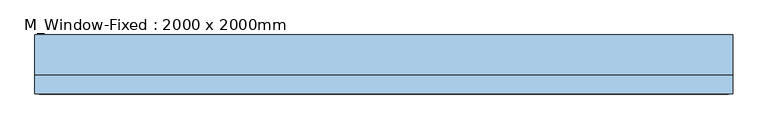
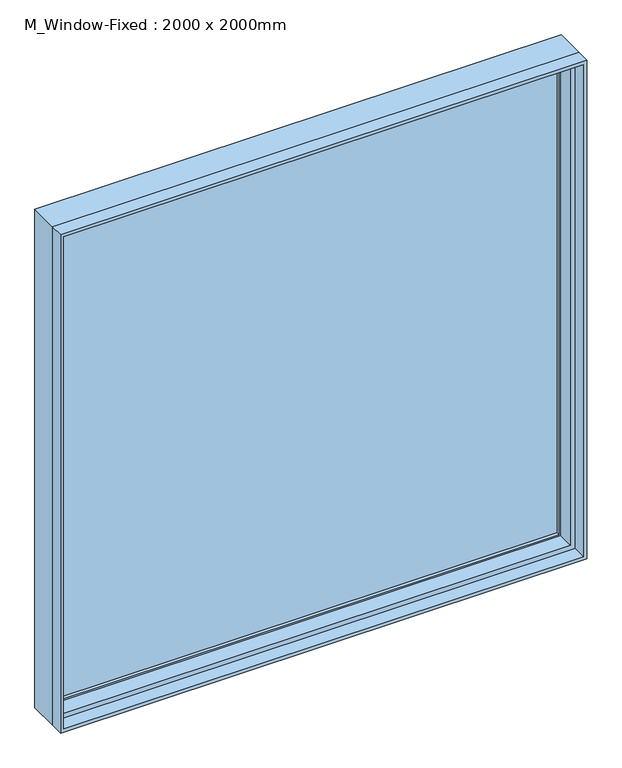
"""IFC4 building model written with IfcOpenShell, lengths in millimetres: window geometry, M_Window-Fixed : 2000 x 2000mm."""

from ifc_helpers import new_model, si_unit, frame, origin, place, context, project, spatial, polyline, outline, extrude, faceted_brep, source, transform, mapped, element, save


def m_window_fixed_2000_x_2000mm_1dfd0f54(model_context):
    return source(origin(), model_context, "Body", "SolidModel", [
        faceted_brep([(1000.0, -20.25, 2900.0), (1000.0, 94.05, 2900.0), (-1000.0, 94.05, 2900.0), (-1000.0, -20.25, 2900.0), (-1000.0, 94.05, 900.0), (-1000.0, -20.25, 900.0), (1000.0, 94.05, 900.0), (1000.0, -20.25, 900.0), (968.25, -20.25, 2868.25), (968.25, -20.25, 931.75), (-968.25, -20.25, 931.75), (-968.25, -20.25, 2868.25), (-987.3, 94.05, 2887.3), (-987.3, 94.05, 912.7), (987.3, 94.05, 912.7), (987.3, 94.05, 2887.3), (968.25, 43.25, 2868.25), (-968.25, 43.25, 2868.25), (987.3, 43.25, 2887.3), (-987.3, 43.25, 2887.3), (-968.25, 43.25, 931.75), (-987.3, 43.25, 912.7), (968.25, 43.25, 931.75), (987.3, 43.25, 912.7)], [[[0, 1, 2, 3]], [[3, 2, 4, 5]], [[5, 4, 6, 7]], [[3, 5, 7, 0], [8, 9, 10, 11]], [[7, 6, 1, 0]], [[1, 6, 4, 2], [12, 13, 14, 15]], [[16, 8, 11, 17]], [[15, 18, 19, 12]], [[17, 11, 10, 20]], [[12, 19, 21, 13]], [[20, 10, 9, 22]], [[13, 21, 23, 14]], [[22, 9, 8, 16]], [[18, 23, 21, 19], [17, 20, 22, 16]], [[14, 23, 18, 15]]]),
        extrude(outline(polyline([(2900.0, -1000.0), (900.0, -1000.0), (900.0, 1000.0), (2900.0, 1000.0), (2900.0, -1000.0)]), holes=[polyline([(2887.3, 987.3), (912.7, 987.3), (912.7, -987.3), (2887.3, -987.3), (2887.3, 987.3)])]), frame((0.0, -75.0, 0.0), z_axis=(0.0, 1.0, 0.0), x_axis=(0.0, 0.0, 1.0)), (0.0, 0.0, 1.0), 54.75),
        extrude(outline(polyline([(912.7, 987.3), (2887.3, 987.3), (2887.3, -987.3), (912.7, -987.3), (912.7, 987.3)]), holes=[polyline([(938.1, -961.9), (2861.9, -961.9), (2861.9, 961.9), (938.1, 961.9), (938.1, -961.9)])]), frame((0.0, 43.25, 0.0), z_axis=(0.0, 1.0, 0.0), x_axis=(0.0, 0.0, 1.0)), (0.0, 0.0, 1.0), 44.45),
        extrude(outline(polyline([(961.9, 75.0), (961.9, 68.65), (-961.9, 68.65), (-961.9, 75.0), (961.9, 75.0)])), frame((0.0, 0.0, 938.1), z_axis=(0.0, 0.0, 1.0), x_axis=(1.0, 0.0, 0.0)), (0.0, 0.0, 1.0), 1923.8),
        extrude(outline(polyline([(-961.9, 55.95), (-961.9, 62.3), (961.9, 62.3), (961.9, 55.95), (-961.9, 55.95)])), frame((0.0, 0.0, 938.1), z_axis=(0.0, 0.0, 1.0), x_axis=(1.0, 0.0, 0.0)), (0.0, 0.0, 1.0), 1923.8),
    ])


if __name__ == "__main__":
    model = new_model("IFC4")
    model_context = context("Model", 3, world=origin())
    ifc_project = project(units=[si_unit("LENGTHUNIT", "METRE", prefix="MILLI")], contexts=[model_context])
    site = spatial("IfcSite", under=ifc_project)
    building = spatial("IfcBuilding", under=site)
    placement = place(None, origin())
    m_window_fixed_2000_x_2000mm_shape = m_window_fixed_2000_x_2000mm_1dfd0f54(model_context)
    element("IfcWindow", 1, ObjectType="M_Window-Fixed : 2000 x 2000mm", at=placement, inside=building, context=model_context, shape_type="MappedRepresentation", body=[
        mapped(m_window_fixed_2000_x_2000mm_shape, transform((0.0, 0.0, 0.0), x_axis=(1.0, 0.0, 0.0), y_axis=(0.0, 1.0, 0.0), z_axis=(0.0, 0.0, 1.0))),
    ])
    save(model, "model.ifc")

# Revit data of these elements
# Type "M_Window-Fixed : 2000 x 2000mm"
#   Type Mark = "40"
#   Fire Rating = "0.5h"
#   Assembly Code = "B2020100"
#   Analytic Construction = "Double glazing - domestic"
#   Window Inset [instance default] = 0 mm
#   Wall Thickness [instance default] = 150 mm
#   Visual Light Transmittance = 0.81
#   Thermal Resistance (R) = 0.319569 (m²·K)/W
#   Solar Heat Gain Coefficient = 0.76
#   Rough Width = 2015 mm
#   Rough Height = 2015 mm
#   Interior Wall Closure [instance default] = 54.75 mm
#   Height = 2000 mm
#   Heat Transfer Coefficient (U) = 3.12929 W/(m²·K)
#   Frame Extension [instance default] = 6.35 mm
#   Exterior Wall Closure [instance default] = 31.75 mm
#   Extension Jamb [instance default] = 54.75 mm
#   Default Sill Height = 900 mm
#   Width = 2000 mm
#   Muntin Visibility = yes
#   Interior Trim Visibility [instance default] = yes
#   Exterior Trim Visibility [instance default] = yes
#   Extension Jamb Visibility [instance default] = yes
#   Muntin Pattern = M_Muntin Pattern_2x2 : M_Muntin Pattern_2x2
#   Interior Trim Material = Wood - Stained
#   Interior Trim = M_Trim-Window-Interior-Flat : Picture Frame
#   Interior Frame Material = Wood - Stained
#   Glass Panel Material = Glass
#   Exterior Trim Material = Clad - White
#   Exterior Trim = M_Trim-Window-Exterior-Flat : with Sill
#   Exterior Frame Material = Clad - White
#   Wall Closure = (empty or 0)
# Element 1 (IfcWindow, "M_Window-Fixed : 2000 x 2000mm")
#   Materials on its faces: "Wood - Stained", "Glass", "Clad - White"
# Materials
#   "Wood - Stained": class "Wood", colour RGB 173 132 96, transparency 0, Cost = 0
#   "Glass": class "Glass", colour RGB 245 245 243, transparency 1, Description = "Soda Lime Glass", Cost = 0
#   "Clad - White": class "Wood", colour RGB 245 245 243, transparency 0, Cost = 0
